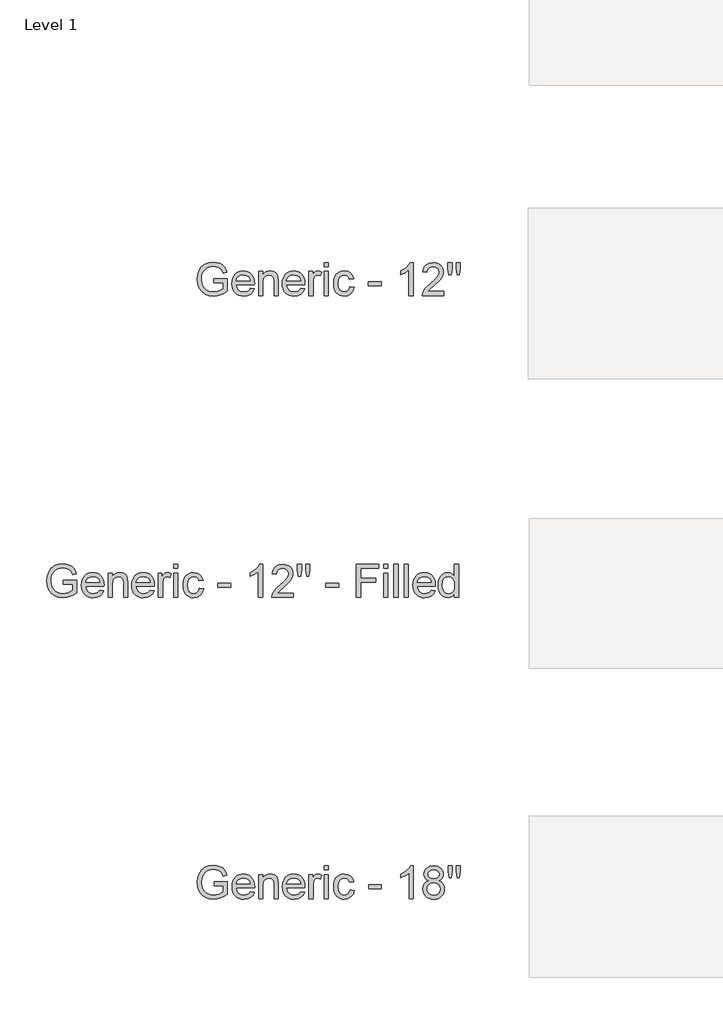
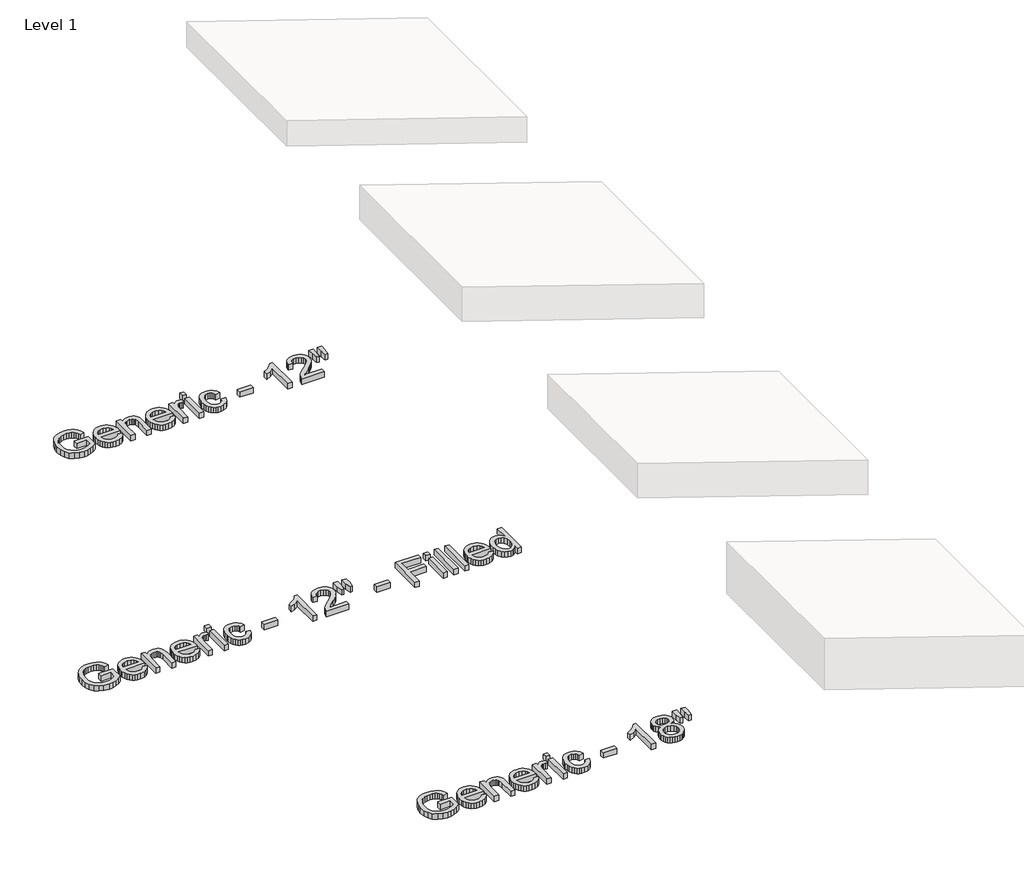
# One storey, part 4 of 42: 3 proxies.
"""IFC4 building model written with IfcOpenShell, lengths in millimetres."""

from ifc_helpers import new_model, si_unit, origin, origin_with_axes, place, context, project, spatial, polyline, outline, extrude, element, save

model = new_model("IFC4")

# Units and contexts
model_context = context("Model", 3, world=origin())
ifc_project = project(units=[si_unit("LENGTHUNIT", "METRE", prefix="MILLI")], contexts=[model_context])

# Site, building, storey
site = spatial("IfcSite", under=ifc_project)
building = spatial("IfcBuilding", under=site)
storey = spatial("IfcBuildingStorey", under=building, Name="Level 1", Elevation=0.0)

# Proxies
placement = place(None, origin())
element("IfcBuildingElementProxy", 1, Name="8\" Arial", ObjectType="8\" Arial", at=placement, inside=storey, context=model_context, shape_type="SweptSolid", body=[
    extrude(outline(polyline([(-15702.4339019, -8427.0985028), (-15702.4339019, -8389.027616), (-15578.7035199, -8389.027616), (-15578.7035199, -8502.8684903), (-15608.7717129, -8523.781453), (-15639.7879603, -8538.7830182), (-15671.6779047, -8547.8174181), (-15704.3671891, -8550.8288847), (-15747.0761063, -8546.0421399), (-15785.6767881, -8531.6819055), (-15817.7433309, -8508.2500927), (-15840.849831, -8476.2486124), (-15854.8196901, -8437.8617076), (-15859.4763098, -8395.2736209), (-15854.8382794, -8352.3788107), (-15840.9241882, -8312.4768779), (-15818.3103045, -8279.0068429), (-15803.9570411, -8265.9734198), (-15787.5728967, -8255.4077263), (-15750.1340461, -8241.4099833), (-15707.4158343, -8236.744069), (-15676.0556849, -8239.4488121), (-15647.8557166, -8247.5630417), (-15624.1078856, -8260.5011946), (-15606.1041484, -8277.6777079), (-15592.7849148, -8299.9198056), (-15583.0905948, -8328.0547114), (-15618.1871935, -8337.9442191), (-15626.0225835, -8317.8770696), (-15635.5495999, -8302.7360846), (-15648.1531454, -8291.3222543), (-15665.2181229, -8282.4365688), (-15685.564112, -8276.720359), (-15708.0106919, -8274.8149557), (-15734.2866677, -8276.8690734), (-15756.751837, -8283.0314264), (-15775.3225479, -8292.5305588), (-15789.9151485, -8304.5950146), (-15809.5082709, -8333.9289303), (-15818.431135, -8362.6679883), (-15821.405423, -8393.7121196), (-15817.8269827, -8430.119264), (-15807.0916619, -8460.0759213), (-15789.5247732, -8483.3683144), (-15765.4516295, -8499.7826664), (-15737.2795451, -8509.5141651), (-15707.4158343, -8512.757998), (-15681.046912, -8510.313505), (-15655.3286152, -8502.9800261), (-15632.9935711, -8492.8767414), (-15616.7744067, -8482.1228313), (-15616.7744067, -8427.0985028), (-15702.4339019, -8427.0985028)])), origin_with_axes(), (0.0, 0.0, 1.0), 50.8),
    extrude(outline(polyline([(-15365.0009251, -8479.445972), (-15327.6736104, -8484.2048329), (-15341.122969, -8512.3304441), (-15362.5843161, -8533.3549426), (-15391.5743297, -8546.4603992), (-15427.6096881, -8550.8288847), (-15451.2320413, -8548.9443944), (-15472.2797764, -8543.2909235), (-15490.7528935, -8533.868472), (-15506.6513924, -8520.6770398), (-15519.4361836, -8504.0837658), (-15528.5681773, -8484.4557884), (-15534.0473736, -8461.7931079), (-15535.8737723, -8436.095724), (-15534.0287843, -8409.5269668), (-15528.4938201, -8386.1090959), (-15519.2688799, -8365.8421114), (-15506.3539636, -8348.7260132), (-15490.4972906, -8335.1279401), (-15472.4470801, -8325.4150308), (-15452.2033322, -8319.5872852), (-15429.7660469, -8317.6447033), (-15408.0514206, -8319.5826379), (-15388.4141487, -8325.3964415), (-15370.854231, -8335.0861142), (-15355.3716676, -8348.651656), (-15342.7332672, -8365.7305756), (-15333.7058383, -8385.9603815), (-15328.2893809, -8409.3410738), (-15326.4838951, -8435.8726524), (-15326.7069667, -8446.1339461), (-15497.8028856, -8446.1339461), (-15491.2129786, -8474.6313433), (-15475.9046899, -8495.5814846), (-15453.8113067, -8508.4638696), (-15426.8661161, -8512.757998), (-15406.6037789, -8510.7689428), (-15389.5388013, -8504.8017775), (-15375.6711834, -8494.4847159), (-15365.0009251, -8479.445972)]), holes=[polyline([(-15497.8028856, -8408.0630594), (-15364.5547819, -8408.0630594), (-15369.704018, -8387.9494366), (-15379.798008, -8373.5613183), (-15401.9936325, -8360.1770221), (-15429.9147613, -8355.7155901), (-15455.5772902, -8359.2754411), (-15476.7969764, -8369.954994), (-15491.547586, -8386.6017123), (-15497.8028856, -8408.0630594)])]), origin_with_axes(), (0.0, 0.0, 1.0), 50.8),
    extrude(outline(polyline([(-15288.4130084, -8546.0700239), (-15288.4130084, -8322.4035642), (-15250.3421216, -8322.4035642), (-15250.3421216, -8353.6335885), (-15237.1158345, -8337.8884512), (-15221.2312775, -8326.6419246), (-15202.6884506, -8319.8940086), (-15181.4873538, -8317.6447033), (-15162.7214552, -8319.4571601), (-15145.5356472, -8324.8945304), (-15131.2032968, -8333.2783048), (-15120.997771, -8343.9299738), (-15109.5839407, -8371.9254598), (-15107.5762963, -8408.7322742), (-15107.5762963, -8546.0700239), (-15145.647183, -8546.0700239), (-15145.647183, -8413.862921), (-15150.0342579, -8380.1791091), (-15156.1036644, -8370.1501817), (-15165.5377342, -8362.3705595), (-15177.630074, -8357.3793324), (-15191.6742903, -8355.7155901), (-15213.9721558, -8359.4520394), (-15232.9797153, -8370.6613874), (-15240.575768, -8379.8119704), (-15246.00152, -8392.3179221), (-15250.3421216, -8427.3959316), (-15250.3421216, -8546.0700239), (-15288.4130084, -8546.0700239)])), origin_with_axes(), (0.0, 0.0, 1.0), 50.8),
    extrude(outline(polyline([(-14898.6325623, -8479.445972), (-14861.3052476, -8484.2048329), (-14874.7546062, -8512.3304441), (-14896.2159533, -8533.3549426), (-14925.2059669, -8546.4603992), (-14961.2413253, -8550.8288847), (-14984.8636785, -8548.9443944), (-15005.9114136, -8543.2909235), (-15024.3845307, -8533.868472), (-15040.2830296, -8520.6770398), (-15053.0678208, -8504.0837658), (-15062.1998146, -8484.4557884), (-15067.6790108, -8461.7931079), (-15069.5054095, -8436.095724), (-15067.6604215, -8409.5269668), (-15062.1254574, -8386.1090959), (-15052.9005171, -8365.8421114), (-15039.9856008, -8348.7260132), (-15024.1289278, -8335.1279401), (-15006.0787173, -8325.4150308), (-14985.8349694, -8319.5872852), (-14963.3976841, -8317.6447033), (-14941.6830579, -8319.5826379), (-14922.0457859, -8325.3964415), (-14904.4858682, -8335.0861142), (-14889.0033048, -8348.651656), (-14876.3649044, -8365.7305756), (-14867.3374755, -8385.9603815), (-14861.9210181, -8409.3410738), (-14860.1155323, -8435.8726524), (-14860.338604, -8446.1339461), (-15031.4345228, -8446.1339461), (-15024.8446158, -8474.6313433), (-15009.5363272, -8495.5814846), (-14987.4429439, -8508.4638696), (-14960.4977533, -8512.757998), (-14940.2354161, -8510.7689428), (-14923.1704385, -8504.8017775), (-14909.3028206, -8494.4847159), (-14898.6325623, -8479.445972)]), holes=[polyline([(-15031.4345228, -8408.0630594), (-14898.1864191, -8408.0630594), (-14903.3356553, -8387.9494366), (-14913.4296453, -8373.5613183), (-14935.6252697, -8360.1770221), (-14963.5463985, -8355.7155901), (-14989.2089274, -8359.2754411), (-15010.4286136, -8369.954994), (-15025.1792233, -8386.6017123), (-15031.4345228, -8408.0630594)])]), origin_with_axes(), (0.0, 0.0, 1.0), 50.8),
    extrude(outline(polyline([(-14822.0446456, -8546.0700239), (-14822.0446456, -8322.4035642), (-14788.7326197, -8322.4035642), (-14788.7326197, -8355.4925185), (-14776.426503, -8336.3083607), (-14765.0870299, -8325.0060662), (-14753.7103781, -8319.485044), (-14741.2927256, -8317.6447033), (-14722.3316395, -8320.5818128), (-14703.0731245, -8329.393141), (-14715.7882058, -8363.5230962), (-14729.1725019, -8357.6674666), (-14742.556798, -8355.7155901), (-14753.9241551, -8357.5931094), (-14764.0832076, -8363.2256674), (-14772.2903837, -8372.18571), (-14777.8021112, -8384.0456835), (-14782.4308469, -8405.3118429), (-14783.9737588, -8428.5112896), (-14783.9737588, -8546.0700239), (-14822.0446456, -8546.0700239)])), origin_with_axes(), (0.0, 0.0, 1.0), 50.8),
    extrude(outline(polyline([(-14679.2788202, -8279.5738166), (-14679.2788202, -8241.5029298), (-14641.2079335, -8241.5029298), (-14641.2079335, -8279.5738166), (-14679.2788202, -8279.5738166)])), origin_with_axes(), (0.0, 0.0, 1.0), 50.8),
    extrude(outline(polyline([(-14679.2788202, -8546.0700239), (-14679.2788202, -8322.4035642), (-14641.2079335, -8322.4035642), (-14641.2079335, -8546.0700239), (-14679.2788202, -8546.0700239)])), origin_with_axes(), (0.0, 0.0, 1.0), 50.8),
    extrude(outline(polyline([(-14441.335778, -8465.1693895), (-14403.2648912, -8469.9282504), (-14413.8793816, -8503.7886606), (-14433.8257007, -8529.3768323), (-14461.2263292, -8545.4658716), (-14494.2037477, -8550.8288847), (-14515.5558826, -8548.9583364), (-14534.7005381, -8543.3466914), (-14551.6377143, -8533.9939497), (-14566.367411, -8520.9001114), (-14578.2901234, -8504.3114847), (-14586.8063465, -8484.4743777), (-14591.9160804, -8461.3887906), (-14593.619325, -8435.0547232), (-14590.7100996, -8401.1757237), (-14581.9824231, -8371.813924), (-14567.296876, -8348.1032717), (-14546.5140384, -8331.1777139), (-14521.6508494, -8321.027956), (-14494.7242481, -8317.6447033), (-14462.5554642, -8322.2920284), (-14436.8371674, -8336.2340035), (-14418.3872869, -8358.7270567), (-14408.0237521, -8389.027616), (-14446.0946388, -8393.7864768), (-14453.0005639, -8377.1769371), (-14463.754474, -8365.2704904), (-14477.7615117, -8358.1043152), (-14494.4268193, -8355.7155901), (-14519.0297581, -8360.418683), (-14538.5578179, -8374.5279619), (-14551.3007832, -8398.8055879), (-14555.5484383, -8434.0137224), (-14551.3937297, -8469.6958841), (-14538.9296039, -8494.057162), (-14519.7547408, -8508.082789), (-14495.4678201, -8512.757998), (-14475.7538673, -8509.8394778), (-14459.5904708, -8501.0839175), (-14447.8327384, -8486.2682452), (-14441.335778, -8465.1693895)])), origin_with_axes(), (0.0, 0.0, 1.0), 50.8),
    extrude(outline(polyline([(-14270.0167876, -8455.6516678), (-14270.0167876, -8417.5807811), (-14151.0452665, -8417.5807811), (-14151.0452665, -8455.6516678), (-14270.0167876, -8455.6516678)])), origin_with_axes(), (0.0, 0.0, 1.0), 50.8),
    extrude(outline(polyline([(-13855.9958941, -8546.0700239), (-13894.0667809, -8546.0700239), (-13894.0667809, -8308.7218392), (-13930.1300232, -8334.4122521), (-13970.2085544, -8353.6335885), (-13970.2085544, -8317.6447033), (-13940.307665, -8301.3790657), (-13914.4034752, -8282.0276042), (-13893.983129, -8261.4492489), (-13880.5337703, -8241.5029298), (-13855.9958941, -8241.5029298), (-13855.9958941, -8546.0700239)])), origin_with_axes(), (0.0, 0.0, 1.0), 50.8),
    extrude(outline(polyline([(-13570.4642434, -8507.9991371), (-13570.4642434, -8546.0700239), (-13770.3363989, -8546.0700239), (-13766.2467528, -8519.821932), (-13756.8591563, -8499.3086393), (-13743.1216634, -8479.4087934), (-13723.2497015, -8458.5794826), (-13695.4586978, -8435.2777948), (-13654.3763444, -8398.7869986), (-13629.7269324, -8371.8511026), (-13617.4022263, -8349.9900856), (-13613.293991, -8328.7239262), (-13617.1698601, -8309.6605989), (-13628.7974674, -8293.8132205), (-13646.6710795, -8283.1336675), (-13669.2849631, -8279.5738166), (-13693.0327941, -8283.0500157), (-13711.4826745, -8293.4786131), (-13723.3891213, -8310.0416796), (-13727.5066513, -8331.9212859), (-13765.577538, -8327.162425), (-13762.3034975, -8307.5088874), (-13756.3479505, -8290.3370214), (-13747.7108969, -8275.6468269), (-13736.3923368, -8263.438304), (-13722.6525203, -8253.8415778), (-13706.7516976, -8246.9867734), (-13668.4670339, -8241.5029298), (-13648.0629533, -8243.0272524), (-13629.9035307, -8247.6002203), (-13613.9887661, -8255.2218333), (-13600.3186595, -8265.8920916), (-13589.3393541, -8278.8209499), (-13581.4969931, -8293.2183629), (-13576.7915764, -8309.0843306), (-13575.2231042, -8326.418853), (-13576.9147306, -8344.6270725), (-13581.9896095, -8362.5192739), (-13590.9961254, -8380.7181988), (-13604.4826627, -8399.8465887), (-13625.9811884, -8422.683544), (-13659.0236694, -8452.008165), (-13702.8200606, -8488.6290863), (-13719.996574, -8507.9991371), (-13570.4642434, -8507.9991371)])), origin_with_axes(), (0.0, 0.0, 1.0), 50.8),
    extrude(outline(polyline([(-13523.0987066, -8350.9567292), (-13532.3933566, -8292.1401835), (-13532.3933566, -8241.5029298), (-13494.3224699, -8241.5029298), (-13494.3224699, -8292.1401835), (-13502.6504764, -8350.9567292), (-13523.0987066, -8350.9567292)])), origin_with_axes(), (0.0, 0.0, 1.0), 50.8),
    extrude(outline(polyline([(-13447.1800046, -8350.9567292), (-13456.2515831, -8292.1401835), (-13456.2515831, -8241.5029298), (-13418.1806964, -8241.5029298), (-13418.1806964, -8292.1401835), (-13427.1035605, -8350.9567292), (-13447.1800046, -8350.9567292)])), origin_with_axes(), (0.0, 0.0, 1.0), 50.8),
])
element("IfcBuildingElementProxy", 2, Name="8\" Arial", ObjectType="8\" Arial", at=placement, inside=storey, context=model_context, shape_type="SweptSolid", body=[
    extrude(outline(polyline([(-17098.2012997, -11224.4993034), (-17098.2012997, -11186.4284167), (-16974.4709177, -11186.4284167), (-16974.4709177, -11300.2692909), (-17004.5391107, -11321.1822536), (-17035.5553581, -11336.1838189), (-17067.4453025, -11345.2182188), (-17100.1345869, -11348.2296854), (-17142.843504, -11343.4429406), (-17181.4441859, -11329.0827062), (-17213.5107287, -11305.6508933), (-17236.6172288, -11273.6494131), (-17250.5870879, -11235.2625082), (-17255.2437075, -11192.6744215), (-17250.6056772, -11149.7796114), (-17236.691586, -11109.8776785), (-17214.0777023, -11076.4076436), (-17199.7244389, -11063.3742205), (-17183.3402945, -11052.808527), (-17145.9014439, -11038.810784), (-17103.1832321, -11034.1448696), (-17071.8230827, -11036.8496128), (-17043.6231144, -11044.9638423), (-17019.8752834, -11057.9019952), (-17001.8715462, -11075.0785086), (-16988.5523126, -11097.3206063), (-16978.8579925, -11125.4555121), (-17013.9545913, -11135.3450198), (-17021.7899813, -11115.2778702), (-17031.3169976, -11100.1368852), (-17043.9205432, -11088.7230549), (-17060.9855207, -11079.8373695), (-17081.3315098, -11074.1211597), (-17103.7780897, -11072.2157564), (-17130.0540655, -11074.2698741), (-17152.5192348, -11080.4322271), (-17171.0899457, -11089.9313595), (-17185.6825463, -11101.9958153), (-17205.2756687, -11131.3297309), (-17214.1985328, -11160.068789), (-17217.1728208, -11191.1129203), (-17213.5943805, -11227.5200647), (-17202.8590597, -11257.4767219), (-17185.292171, -11280.769115), (-17161.2190273, -11297.1834671), (-17133.0469428, -11306.9149657), (-17103.1832321, -11310.1587986), (-17076.8143098, -11307.7143057), (-17051.096013, -11300.3808267), (-17028.7609689, -11290.2775421), (-17012.5418045, -11279.5236319), (-17012.5418045, -11224.4993034), (-17098.2012997, -11224.4993034)])), origin_with_axes(), (0.0, 0.0, 1.0), 50.8),
    extrude(outline(polyline([(-16760.7683229, -11276.8467727), (-16723.4410081, -11281.6056336), (-16736.8903668, -11309.7312447), (-16758.3517139, -11330.7557432), (-16787.3417275, -11343.8611998), (-16823.3770859, -11348.2296854), (-16846.9994391, -11346.3451951), (-16868.0471742, -11340.6917242), (-16886.5202912, -11331.2692726), (-16902.4187902, -11318.0778405), (-16915.2035814, -11301.4845664), (-16924.3355751, -11281.8565891), (-16929.8147714, -11259.1939085), (-16931.6411701, -11233.4965247), (-16929.7961821, -11206.9277674), (-16924.2612179, -11183.5098965), (-16915.0362777, -11163.242912), (-16902.1213614, -11146.1268139), (-16886.2646884, -11132.5287408), (-16868.2144779, -11122.8158315), (-16847.97073, -11116.9880859), (-16825.5334447, -11115.045504), (-16803.8188184, -11116.9834385), (-16784.1815465, -11122.7972422), (-16766.6216288, -11132.4869149), (-16751.1390654, -11146.0524567), (-16738.5006649, -11163.1313762), (-16729.473236, -11183.3611821), (-16724.0567787, -11206.7418744), (-16722.2512929, -11233.2734531), (-16722.4743645, -11243.5347468), (-16893.5702833, -11243.5347468), (-16886.9803764, -11272.032144), (-16871.6720877, -11292.9822853), (-16849.5787045, -11305.8646703), (-16822.6335139, -11310.1587986), (-16802.3711767, -11308.1697435), (-16785.3061991, -11302.2025782), (-16771.4385812, -11291.8855166), (-16760.7683229, -11276.8467727)]), holes=[polyline([(-16893.5702833, -11205.46386), (-16760.3221797, -11205.46386), (-16765.4714158, -11185.3502373), (-16775.5654058, -11170.9621189), (-16797.7610302, -11157.5778228), (-16825.6821591, -11153.1163907), (-16851.344688, -11156.6762417), (-16872.5643741, -11167.3557947), (-16887.3149838, -11184.002513), (-16893.5702833, -11205.46386)])]), origin_with_axes(), (0.0, 0.0, 1.0), 50.8),
    extrude(outline(polyline([(-16684.1804062, -11343.4708245), (-16684.1804062, -11119.8043648), (-16646.1095194, -11119.8043648), (-16646.1095194, -11151.0343891), (-16632.8832323, -11135.2892519), (-16616.9986753, -11124.0427253), (-16598.4558484, -11117.2948093), (-16577.2547516, -11115.045504), (-16558.488853, -11116.8579608), (-16541.303045, -11122.2953311), (-16526.9706946, -11130.6791054), (-16516.7651688, -11141.3307744), (-16505.3513385, -11169.3262605), (-16503.3436941, -11206.1330748), (-16503.3436941, -11343.4708245), (-16541.4145808, -11343.4708245), (-16541.4145808, -11211.2637217), (-16545.8016557, -11177.5799098), (-16551.8710622, -11167.5509823), (-16561.305132, -11159.7713602), (-16573.3974718, -11154.7801331), (-16587.4416881, -11153.1163907), (-16609.7395536, -11156.8528401), (-16628.747113, -11168.0621881), (-16636.3431658, -11177.2127711), (-16641.7689178, -11189.7187228), (-16646.1095194, -11224.7967322), (-16646.1095194, -11343.4708245), (-16684.1804062, -11343.4708245)])), origin_with_axes(), (0.0, 0.0, 1.0), 50.8),
    extrude(outline(polyline([(-16294.3999601, -11276.8467727), (-16257.0726453, -11281.6056336), (-16270.522004, -11309.7312447), (-16291.9833511, -11330.7557432), (-16320.9733647, -11343.8611998), (-16357.0087231, -11348.2296854), (-16380.6310763, -11346.3451951), (-16401.6788114, -11340.6917242), (-16420.1519285, -11331.2692726), (-16436.0504274, -11318.0778405), (-16448.8352186, -11301.4845664), (-16457.9672123, -11281.8565891), (-16463.4464086, -11259.1939085), (-16465.2728073, -11233.4965247), (-16463.4278193, -11206.9277674), (-16457.8928551, -11183.5098965), (-16448.6679149, -11163.242912), (-16435.7529986, -11146.1268139), (-16419.8963256, -11132.5287408), (-16401.8461151, -11122.8158315), (-16381.6023672, -11116.9880859), (-16359.1650819, -11115.045504), (-16337.4504556, -11116.9834385), (-16317.8131837, -11122.7972422), (-16300.253266, -11132.4869149), (-16284.7707026, -11146.0524567), (-16272.1323021, -11163.1313762), (-16263.1048733, -11183.3611821), (-16257.6884159, -11206.7418744), (-16255.8829301, -11233.2734531), (-16256.1060017, -11243.5347468), (-16427.2019205, -11243.5347468), (-16420.6120136, -11272.032144), (-16405.3037249, -11292.9822853), (-16383.2103417, -11305.8646703), (-16356.2651511, -11310.1587986), (-16336.0028139, -11308.1697435), (-16318.9378363, -11302.2025782), (-16305.0702184, -11291.8855166), (-16294.3999601, -11276.8467727)]), holes=[polyline([(-16427.2019205, -11205.46386), (-16293.9538169, -11205.46386), (-16299.103053, -11185.3502373), (-16309.197043, -11170.9621189), (-16331.3926674, -11157.5778228), (-16359.3137963, -11153.1163907), (-16384.9763252, -11156.6762417), (-16406.1960113, -11167.3557947), (-16420.946621, -11184.002513), (-16427.2019205, -11205.46386)])]), origin_with_axes(), (0.0, 0.0, 1.0), 50.8),
    extrude(outline(polyline([(-16217.8120434, -11343.4708245), (-16217.8120434, -11119.8043648), (-16184.5000175, -11119.8043648), (-16184.5000175, -11152.8933191), (-16172.1939007, -11133.7091614), (-16160.8544276, -11122.4068669), (-16149.4777759, -11116.8858447), (-16137.0601234, -11115.045504), (-16118.0990372, -11117.9826134), (-16098.8405223, -11126.7939417), (-16111.5556036, -11160.9238968), (-16124.9398997, -11155.0682673), (-16138.3241958, -11153.1163907), (-16149.6915529, -11154.9939101), (-16159.8506054, -11160.626468), (-16168.0577815, -11169.5865107), (-16173.569509, -11181.4464842), (-16178.1982447, -11202.7126436), (-16179.7411566, -11225.9120902), (-16179.7411566, -11343.4708245), (-16217.8120434, -11343.4708245)])), origin_with_axes(), (0.0, 0.0, 1.0), 50.8),
    extrude(outline(polyline([(-16075.046218, -11076.9746172), (-16075.046218, -11038.9037305), (-16036.9753313, -11038.9037305), (-16036.9753313, -11076.9746172), (-16075.046218, -11076.9746172)])), origin_with_axes(), (0.0, 0.0, 1.0), 50.8),
    extrude(outline(polyline([(-16075.046218, -11343.4708245), (-16075.046218, -11119.8043648), (-16036.9753313, -11119.8043648), (-16036.9753313, -11343.4708245), (-16075.046218, -11343.4708245)])), origin_with_axes(), (0.0, 0.0, 1.0), 50.8),
    extrude(outline(polyline([(-15837.1031758, -11262.5701902), (-15799.032289, -11267.329051), (-15809.6467794, -11301.1894613), (-15829.5930985, -11326.777633), (-15856.993727, -11342.8666723), (-15889.9711455, -11348.2296854), (-15911.3232804, -11346.3591371), (-15930.4679359, -11340.7474921), (-15947.405112, -11331.3947504), (-15962.1348088, -11318.3009121), (-15974.0575212, -11301.7122854), (-15982.5737443, -11281.8751784), (-15987.6834782, -11258.7895913), (-15989.3867228, -11232.4555239), (-15986.4774973, -11198.5765243), (-15977.7498209, -11169.2147247), (-15963.0642738, -11145.5040723), (-15942.2814362, -11128.5785145), (-15917.4182472, -11118.4287566), (-15890.4916459, -11115.045504), (-15858.3228619, -11119.692829), (-15832.6045651, -11133.6348042), (-15814.1546847, -11156.1278574), (-15803.7911499, -11186.4284167), (-15841.8620366, -11191.1872775), (-15848.7679616, -11174.5777378), (-15859.5218718, -11162.671291), (-15873.5289095, -11155.5051158), (-15890.1942171, -11153.1163907), (-15914.7971559, -11157.8194837), (-15934.3252157, -11171.9287625), (-15947.068181, -11196.2063886), (-15951.3158361, -11231.4145231), (-15947.1611275, -11267.0966848), (-15934.6970017, -11291.4579626), (-15915.5221386, -11305.4835896), (-15891.2352179, -11310.1587986), (-15871.5212651, -11307.2402785), (-15855.3578686, -11298.4847181), (-15843.6001362, -11283.6690459), (-15837.1031758, -11262.5701902)])), origin_with_axes(), (0.0, 0.0, 1.0), 50.8),
    extrude(outline(polyline([(-15665.7841854, -11253.0524685), (-15665.7841854, -11214.9815817), (-15546.8126643, -11214.9815817), (-15546.8126643, -11253.0524685), (-15665.7841854, -11253.0524685)])), origin_with_axes(), (0.0, 0.0, 1.0), 50.8),
    extrude(outline(polyline([(-15251.7632919, -11343.4708245), (-15289.8341786, -11343.4708245), (-15289.8341786, -11106.1226399), (-15325.897421, -11131.8130527), (-15365.9759522, -11151.0343891), (-15365.9759522, -11115.045504), (-15336.0750628, -11098.7798663), (-15310.170873, -11079.4284049), (-15289.7505268, -11058.8500496), (-15276.3011681, -11038.9037305), (-15251.7632919, -11038.9037305), (-15251.7632919, -11343.4708245)])), origin_with_axes(), (0.0, 0.0, 1.0), 50.8),
    extrude(outline(polyline([(-14966.2316412, -11305.3999378), (-14966.2316412, -11343.4708245), (-15166.1037967, -11343.4708245), (-15162.0141506, -11317.2227327), (-15152.626554, -11296.7094399), (-15138.8890612, -11276.8095941), (-15119.0170993, -11255.9802833), (-15091.2260956, -11232.6785955), (-15050.1437422, -11196.1877993), (-15025.4943301, -11169.2519033), (-15013.1696241, -11147.3908863), (-15009.0613888, -11126.1247269), (-15012.9372579, -11107.0613996), (-15024.5648651, -11091.2140212), (-15042.4384773, -11080.5344682), (-15065.0523609, -11076.9746172), (-15088.8001919, -11080.4508164), (-15107.2500723, -11090.8794138), (-15119.1565191, -11107.4424802), (-15123.2740491, -11129.3220865), (-15161.3449358, -11124.5632257), (-15158.0708953, -11104.9096881), (-15152.1153483, -11087.737822), (-15143.4782947, -11073.0476276), (-15132.1597346, -11060.8391047), (-15118.4199181, -11051.2423785), (-15102.5190954, -11044.387574), (-15064.2344317, -11038.9037305), (-15043.8303511, -11040.4280531), (-15025.6709285, -11045.0010209), (-15009.7561639, -11052.622634), (-14996.0860573, -11063.2928923), (-14985.1067519, -11076.2217506), (-14977.2643908, -11090.6191636), (-14972.5589742, -11106.4851313), (-14970.990502, -11123.8196537), (-14972.6821283, -11142.0278732), (-14977.7570073, -11159.9200746), (-14986.7635232, -11178.1189995), (-15000.2500605, -11197.2473894), (-15021.7485862, -11220.0843446), (-15054.7910672, -11249.4089657), (-15098.5874584, -11286.029887), (-15115.7639718, -11305.3999378), (-14966.2316412, -11305.3999378)])), origin_with_axes(), (0.0, 0.0, 1.0), 50.8),
    extrude(outline(polyline([(-14918.8661043, -11148.3575299), (-14928.1607544, -11089.5409841), (-14928.1607544, -11038.9037305), (-14890.0898677, -11038.9037305), (-14890.0898677, -11089.5409841), (-14898.4178741, -11148.3575299), (-14918.8661043, -11148.3575299)])), origin_with_axes(), (0.0, 0.0, 1.0), 50.8),
    extrude(outline(polyline([(-14842.9474024, -11148.3575299), (-14852.0189809, -11089.5409841), (-14852.0189809, -11038.9037305), (-14813.9480942, -11038.9037305), (-14813.9480942, -11089.5409841), (-14822.8709582, -11148.3575299), (-14842.9474024, -11148.3575299)])), origin_with_axes(), (0.0, 0.0, 1.0), 50.8),
    extrude(outline(polyline([(-14666.423408, -11253.0524685), (-14666.423408, -11214.9815817), (-14547.4518868, -11214.9815817), (-14547.4518868, -11253.0524685), (-14666.423408, -11253.0524685)])), origin_with_axes(), (0.0, 0.0, 1.0), 50.8),
    extrude(outline(polyline([(-14380.8917573, -11343.4708245), (-14380.8917573, -11038.9037305), (-14176.2607409, -11038.9037305), (-14176.2607409, -11076.9746172), (-14342.8208705, -11076.9746172), (-14342.8208705, -11167.3929733), (-14200.0550452, -11167.3929733), (-14200.0550452, -11205.46386), (-14342.8208705, -11205.46386), (-14342.8208705, -11343.4708245), (-14380.8917573, -11343.4708245)])), origin_with_axes(), (0.0, 0.0, 1.0), 50.8),
    extrude(outline(polyline([(-14128.6721325, -11076.9746172), (-14128.6721325, -11038.9037305), (-14090.6012457, -11038.9037305), (-14090.6012457, -11076.9746172), (-14128.6721325, -11076.9746172)])), origin_with_axes(), (0.0, 0.0, 1.0), 50.8),
    extrude(outline(polyline([(-14128.6721325, -11343.4708245), (-14128.6721325, -11119.8043648), (-14090.6012457, -11119.8043648), (-14090.6012457, -11343.4708245), (-14128.6721325, -11343.4708245)])), origin_with_axes(), (0.0, 0.0, 1.0), 50.8),
    extrude(outline(polyline([(-14033.4949156, -11343.4708245), (-14033.4949156, -11038.9037305), (-13995.4240288, -11038.9037305), (-13995.4240288, -11343.4708245), (-14033.4949156, -11343.4708245)])), origin_with_axes(), (0.0, 0.0, 1.0), 50.8),
    extrude(outline(polyline([(-13938.3176987, -11343.4708245), (-13938.3176987, -11038.9037305), (-13900.2468119, -11038.9037305), (-13900.2468119, -11343.4708245), (-13938.3176987, -11343.4708245)])), origin_with_axes(), (0.0, 0.0, 1.0), 50.8),
    extrude(outline(polyline([(-13686.5442171, -11276.8467727), (-13649.2169024, -11281.6056336), (-13662.6662611, -11309.7312447), (-13684.1276081, -11330.7557432), (-13713.1176217, -11343.8611998), (-13749.1529801, -11348.2296854), (-13772.7753333, -11346.3451951), (-13793.8230684, -11340.6917242), (-13812.2961855, -11331.2692726), (-13828.1946845, -11318.0778405), (-13840.9794757, -11301.4845664), (-13850.1114694, -11281.8565891), (-13855.5906656, -11259.1939085), (-13857.4170643, -11233.4965247), (-13855.5720763, -11206.9277674), (-13850.0371122, -11183.5098965), (-13840.812172, -11163.242912), (-13827.8972557, -11146.1268139), (-13812.0405826, -11132.5287408), (-13793.9903721, -11122.8158315), (-13773.7466243, -11116.9880859), (-13751.3093389, -11115.045504), (-13729.5947127, -11116.9834385), (-13709.9574407, -11122.7972422), (-13692.397523, -11132.4869149), (-13676.9149596, -11146.0524567), (-13664.2765592, -11163.1313762), (-13655.2491303, -11183.3611821), (-13649.832673, -11206.7418744), (-13648.0271872, -11233.2734531), (-13648.2502588, -11243.5347468), (-13819.3461776, -11243.5347468), (-13812.7562707, -11272.032144), (-13797.447982, -11292.9822853), (-13775.3545987, -11305.8646703), (-13748.4094081, -11310.1587986), (-13728.1470709, -11308.1697435), (-13711.0820934, -11302.2025782), (-13697.2144754, -11291.8855166), (-13686.5442171, -11276.8467727)]), holes=[polyline([(-13819.3461776, -11205.46386), (-13686.0980739, -11205.46386), (-13691.2473101, -11185.3502373), (-13701.3413001, -11170.9621189), (-13723.5369245, -11157.5778228), (-13751.4580533, -11153.1163907), (-13777.1205822, -11156.6762417), (-13798.3402684, -11167.3557947), (-13813.0908781, -11184.002513), (-13819.3461776, -11205.46386)])]), origin_with_axes(), (0.0, 0.0, 1.0), 50.8),
    extrude(outline(polyline([(-13471.9493359, -11343.4708245), (-13471.9493359, -11307.5562966), (-13483.3399296, -11325.3509042), (-13497.1378377, -11338.0613382), (-13513.3430601, -11345.6875986), (-13531.9555969, -11348.2296854), (-13556.5678303, -11344.5490039), (-13579.0980621, -11333.5069596), (-13598.1706841, -11315.8750084), (-13612.410088, -11292.4246063), (-13621.2771842, -11264.1038074), (-13624.2328829, -11231.8606663), (-13621.5095505, -11200.0171951), (-13613.339553, -11171.2595477), (-13599.7321853, -11147.2235826), (-13580.6967419, -11129.5451581), (-13557.6738937, -11118.6704175), (-13532.1043113, -11115.045504), (-13513.4778325, -11117.6387114), (-13497.0077126, -11125.4183335), (-13483.0471481, -11137.3433695), (-13471.9493359, -11152.3728187), (-13471.9493359, -11038.9037305), (-13433.8784492, -11038.9037305), (-13433.8784492, -11343.4708245), (-13471.9493359, -11343.4708245)]), holes=[polyline([(-13586.1619962, -11231.7119519), (-13581.8678679, -11266.1486305), (-13568.9854828, -11290.6400334), (-13550.2660576, -11305.2791073), (-13528.4608084, -11310.1587986), (-13506.664854, -11305.5021789), (-13488.4194559, -11291.5323199), (-13476.0668659, -11267.9889712), (-13471.9493359, -11234.6118827), (-13476.1412231, -11198.1210865), (-13488.7168847, -11172.8210489), (-13507.4270153, -11158.0425553), (-13530.0223097, -11153.1163907), (-13552.0506304, -11157.8473676), (-13570.1008408, -11172.0402983), (-13582.1467074, -11196.4201655), (-13586.1619962, -11231.7119519)])]), origin_with_axes(), (0.0, 0.0, 1.0), 50.8),
])
element("IfcBuildingElementProxy", 3, Name="8\" Arial", ObjectType="8\" Arial", at=placement, inside=storey, context=model_context, shape_type="SweptSolid", body=[
    extrude(outline(polyline([(-15701.6648928, -14020.780444), (-15701.6648928, -13982.7095572), (-15577.9345108, -13982.7095572), (-15577.9345108, -14096.5504315), (-15608.0027038, -14117.4633942), (-15639.0189512, -14132.4649594), (-15670.9088956, -14141.4993593), (-15703.59818, -14144.510826), (-15746.3070971, -14139.7240812), (-15784.907779, -14125.3638468), (-15816.9743218, -14101.9320339), (-15840.0808219, -14069.9305537), (-15854.050681, -14031.5436488), (-15858.7073007, -13988.9555621), (-15854.0692703, -13946.0607519), (-15840.1551791, -13906.1588191), (-15817.5412954, -13872.6887842), (-15803.188032, -13859.6553611), (-15786.8038876, -13849.0896676), (-15749.365037, -13835.0919245), (-15706.6468252, -13830.4260102), (-15675.2866758, -13833.1307534), (-15647.0867075, -13841.2449829), (-15623.3388765, -13854.1831358), (-15605.3351393, -13871.3596492), (-15592.0159057, -13893.6017468), (-15582.3215857, -13921.7366527), (-15617.4181844, -13931.6261604), (-15625.2535744, -13911.5590108), (-15634.7805907, -13896.4180258), (-15647.3841363, -13885.0041955), (-15664.4491138, -13876.11851), (-15684.7951029, -13870.4023002), (-15707.2416828, -13868.496897), (-15733.5176586, -13870.5510146), (-15755.9828279, -13876.7133676), (-15774.5535388, -13886.2125), (-15789.1461394, -13898.2769558), (-15808.7392618, -13927.6108715), (-15817.6621259, -13956.3499296), (-15820.6364139, -13987.3940609), (-15817.0579736, -14023.8012053), (-15806.3226528, -14053.7578625), (-15788.7557641, -14077.0502556), (-15764.6826204, -14093.4646077), (-15736.510536, -14103.1961063), (-15706.6468252, -14106.4399392), (-15680.2779029, -14103.9954462), (-15654.5596061, -14096.6619673), (-15632.224562, -14086.5586827), (-15616.0053976, -14075.8047725), (-15616.0053976, -14020.780444), (-15701.6648928, -14020.780444)])), origin_with_axes(), (0.0, 0.0, 1.0), 50.8),
    extrude(outline(polyline([(-15364.231916, -14073.1279133), (-15326.9046012, -14077.8867741), (-15340.3539599, -14106.0123853), (-15361.815307, -14127.0368838), (-15390.8053206, -14140.1423404), (-15426.840679, -14144.510826), (-15450.4630322, -14142.6263357), (-15471.5107673, -14136.9728647), (-15489.9838844, -14127.5504132), (-15505.8823833, -14114.3589811), (-15518.6671745, -14097.765707), (-15527.7991682, -14078.1377297), (-15533.2783645, -14055.4750491), (-15535.1047632, -14029.7776653), (-15533.2597752, -14003.208908), (-15527.724811, -13979.7910371), (-15518.4998708, -13959.5240526), (-15505.5849545, -13942.4079545), (-15489.7282815, -13928.8098814), (-15471.678071, -13919.096972), (-15451.4343231, -13913.2692264), (-15428.9970378, -13911.3266446), (-15407.2824115, -13913.2645791), (-15387.6451396, -13919.0783827), (-15370.0852219, -13928.7680555), (-15354.6026585, -13942.3335973), (-15341.9642581, -13959.4125168), (-15332.9368292, -13979.6423227), (-15327.5203718, -14003.023015), (-15325.714886, -14029.5545937), (-15325.9379576, -14039.8158874), (-15497.0338765, -14039.8158874), (-15490.4439695, -14068.3132845), (-15475.1356808, -14089.2634258), (-15453.0422976, -14102.1458109), (-15426.097107, -14106.4399392), (-15405.8347698, -14104.4508841), (-15388.7697922, -14098.4837187), (-15374.9021743, -14088.1666571), (-15364.231916, -14073.1279133)]), holes=[polyline([(-15497.0338765, -14001.7450006), (-15363.7857728, -14001.7450006), (-15368.9350089, -13981.6313778), (-15379.0289989, -13967.2432595), (-15401.2246233, -13953.8589634), (-15429.1457522, -13949.3975313), (-15454.8082811, -13952.9573823), (-15476.0279673, -13963.6369353), (-15490.7785769, -13980.2836536), (-15497.0338765, -14001.7450006)])]), origin_with_axes(), (0.0, 0.0, 1.0), 50.8),
    extrude(outline(polyline([(-15287.6439993, -14139.7519651), (-15287.6439993, -13916.0855054), (-15249.5731125, -13916.0855054), (-15249.5731125, -13947.3155297), (-15236.3468254, -13931.5703925), (-15220.4622684, -13920.3238658), (-15201.9194415, -13913.5759499), (-15180.7183447, -13911.3266446), (-15161.9524461, -13913.1391013), (-15144.7666381, -13918.5764716), (-15130.4342877, -13926.960246), (-15120.2287619, -13937.611915), (-15108.8149316, -13965.6074011), (-15106.8072872, -14002.4142154), (-15106.8072872, -14139.7519651), (-15144.8781739, -14139.7519651), (-15144.8781739, -14007.5448623), (-15149.2652488, -13973.8610504), (-15155.3346553, -13963.8321229), (-15164.7687251, -13956.0525008), (-15176.8610649, -13951.0612737), (-15190.9052812, -13949.3975313), (-15213.2031467, -13953.1339807), (-15232.2107062, -13964.3433287), (-15239.8067589, -13973.4939117), (-15245.2325109, -13985.9998634), (-15249.5731125, -14021.0778728), (-15249.5731125, -14139.7519651), (-15287.6439993, -14139.7519651)])), origin_with_axes(), (0.0, 0.0, 1.0), 50.8),
    extrude(outline(polyline([(-14897.8635532, -14073.1279133), (-14860.5362385, -14077.8867741), (-14873.9855971, -14106.0123853), (-14895.4469442, -14127.0368838), (-14924.4369578, -14140.1423404), (-14960.4723162, -14144.510826), (-14984.0946694, -14142.6263357), (-15005.1424045, -14136.9728647), (-15023.6155216, -14127.5504132), (-15039.5140205, -14114.3589811), (-15052.2988117, -14097.765707), (-15061.4308054, -14078.1377297), (-15066.9100017, -14055.4750491), (-15068.7364004, -14029.7776653), (-15066.8914124, -14003.208908), (-15061.3564482, -13979.7910371), (-15052.131508, -13959.5240526), (-15039.2165917, -13942.4079545), (-15023.3599187, -13928.8098814), (-15005.3097082, -13919.096972), (-14985.0659603, -13913.2692264), (-14962.628675, -13911.3266446), (-14940.9140488, -13913.2645791), (-14921.2767768, -13919.0783827), (-14903.7168591, -13928.7680555), (-14888.2342957, -13942.3335973), (-14875.5958953, -13959.4125168), (-14866.5684664, -13979.6423227), (-14861.152009, -14003.023015), (-14859.3465232, -14029.5545937), (-14859.5695948, -14039.8158874), (-15030.6655137, -14039.8158874), (-15024.0756067, -14068.3132845), (-15008.7673181, -14089.2634258), (-14986.6739348, -14102.1458109), (-14959.7287442, -14106.4399392), (-14939.466407, -14104.4508841), (-14922.4014294, -14098.4837187), (-14908.5338115, -14088.1666571), (-14897.8635532, -14073.1279133)]), holes=[polyline([(-15030.6655137, -14001.7450006), (-14897.41741, -14001.7450006), (-14902.5666462, -13981.6313778), (-14912.6606361, -13967.2432595), (-14934.8562606, -13953.8589634), (-14962.7773894, -13949.3975313), (-14988.4399183, -13952.9573823), (-15009.6596045, -13963.6369353), (-15024.4102142, -13980.2836536), (-15030.6655137, -14001.7450006)])]), origin_with_axes(), (0.0, 0.0, 1.0), 50.8),
    extrude(outline(polyline([(-14821.2756365, -14139.7519651), (-14821.2756365, -13916.0855054), (-14787.9636106, -13916.0855054), (-14787.9636106, -13949.1744597), (-14775.6574939, -13929.9903019), (-14764.3180208, -13918.6880074), (-14752.941369, -13913.1669853), (-14740.5237165, -13911.3266446), (-14721.5626303, -13914.263754), (-14702.3041154, -13923.0750823), (-14715.0191967, -13957.2050374), (-14728.4034928, -13951.3494078), (-14741.7877889, -13949.3975313), (-14753.155146, -13951.2750506), (-14763.3141985, -13956.9076086), (-14771.5213746, -13965.8676513), (-14777.0331021, -13977.7276248), (-14781.6618378, -13998.9937842), (-14783.2047497, -14022.1932308), (-14783.2047497, -14139.7519651), (-14821.2756365, -14139.7519651)])), origin_with_axes(), (0.0, 0.0, 1.0), 50.8),
    extrude(outline(polyline([(-14678.5098111, -13873.2557578), (-14678.5098111, -13835.184871), (-14640.4389244, -13835.184871), (-14640.4389244, -13873.2557578), (-14678.5098111, -13873.2557578)])), origin_with_axes(), (0.0, 0.0, 1.0), 50.8),
    extrude(outline(polyline([(-14678.5098111, -14139.7519651), (-14678.5098111, -13916.0855054), (-14640.4389244, -13916.0855054), (-14640.4389244, -14139.7519651), (-14678.5098111, -14139.7519651)])), origin_with_axes(), (0.0, 0.0, 1.0), 50.8),
    extrude(outline(polyline([(-14440.5667689, -14058.8513308), (-14402.4958821, -14063.6101916), (-14413.1103725, -14097.4706019), (-14433.0566916, -14123.0587736), (-14460.4573201, -14139.1478129), (-14493.4347386, -14144.510826), (-14514.7868735, -14142.6402776), (-14533.931529, -14137.0286326), (-14550.8687052, -14127.675891), (-14565.5984019, -14114.5820527), (-14577.5211143, -14097.9934259), (-14586.0373374, -14078.156319), (-14591.1470713, -14055.0707318), (-14592.8503159, -14028.7366645), (-14589.9410905, -13994.8576649), (-14581.213414, -13965.4958653), (-14566.5278669, -13941.7852129), (-14545.7450293, -13924.8596551), (-14520.8818403, -13914.7098972), (-14493.955239, -13911.3266446), (-14461.7864551, -13915.9739696), (-14436.0681583, -13929.9159447), (-14417.6182778, -13952.408998), (-14407.254743, -13982.7095572), (-14445.3256297, -13987.4684181), (-14452.2315548, -13970.8588784), (-14462.9854649, -13958.9524316), (-14476.9925026, -13951.7862564), (-14493.6578102, -13949.3975313), (-14518.260749, -13954.1006243), (-14537.7888088, -13968.2099031), (-14550.5317741, -13992.4875291), (-14554.7794292, -14027.6956637), (-14550.6247206, -14063.3778253), (-14538.1605948, -14087.7391032), (-14518.9857317, -14101.7647302), (-14494.698811, -14106.4399392), (-14474.9848582, -14103.5214191), (-14458.8214617, -14094.7658587), (-14447.0637293, -14079.9501865), (-14440.5667689, -14058.8513308)])), origin_with_axes(), (0.0, 0.0, 1.0), 50.8),
    extrude(outline(polyline([(-14269.2477785, -14049.3336091), (-14269.2477785, -14011.2627223), (-14150.2762574, -14011.2627223), (-14150.2762574, -14049.3336091), (-14269.2477785, -14049.3336091)])), origin_with_axes(), (0.0, 0.0, 1.0), 50.8),
    extrude(outline(polyline([(-13855.226885, -14139.7519651), (-13893.2977717, -14139.7519651), (-13893.2977717, -13902.4037805), (-13929.3610141, -13928.0941933), (-13969.4395453, -13947.3155297), (-13969.4395453, -13911.3266446), (-13939.5386559, -13895.0610069), (-13913.6344661, -13875.7095454), (-13893.2141199, -13855.1311901), (-13879.7647612, -13835.184871), (-13855.226885, -13835.184871), (-13855.226885, -14139.7519651)])), origin_with_axes(), (0.0, 0.0, 1.0), 50.8),
    extrude(outline(polyline([(-13709.3380572, -13972.0021203), (-13729.7212249, -13961.9638982), (-13744.0256913, -13948.3565305), (-13752.4745283, -13931.4588567), (-13755.2908072, -13911.5497162), (-13753.75719, -13896.0230032), (-13749.1563382, -13881.7882466), (-13741.4882519, -13868.8454463), (-13730.752931, -13857.1946025), (-13717.4662287, -13847.565345), (-13702.143998, -13840.6873039), (-13665.3929516, -13835.184871), (-13628.4188336, -13840.817429), (-13612.9292992, -13847.8581264), (-13599.4381146, -13857.7151029), (-13588.5076061, -13869.5936657), (-13580.7001, -13882.6991223), (-13576.0155964, -13897.0314727), (-13574.4540951, -13912.590717), (-13577.2331955, -13931.8585266), (-13585.5704967, -13948.4680663), (-13599.558945, -13961.9917822), (-13619.2914872, -13972.0021203), (-13595.8596743, -13984.0758708), (-13578.8039914, -14001.8565364), (-13568.4032779, -14024.4890094), (-13564.9363735, -14051.1181819), (-13566.6558837, -14070.107152), (-13571.8144145, -14087.5160316), (-13580.4119659, -14103.3448207), (-13592.4485377, -14117.5935193), (-13607.2920939, -14129.369841), (-13624.3105982, -14137.7814993), (-13643.5040506, -14142.8284943), (-13664.8724512, -14144.510826), (-13686.2408517, -14142.8215233), (-13705.4343042, -14137.7536153), (-13722.4528085, -14129.3071021), (-13737.2963647, -14117.4819835), (-13749.3329365, -14103.1333674), (-13757.9304879, -14087.1163617), (-13763.0890187, -14069.4309662), (-13764.8085289, -14050.0771811), (-13761.2022047, -14022.4163024), (-13750.383232, -13999.662999), (-13732.9092898, -13982.5980214), (-13709.3380572, -13972.0021203)]), holes=[polyline([(-13717.2199205, -13912.6650742), (-13713.8459625, -13929.2839085), (-13703.7240886, -13942.5566689), (-13687.1517275, -13951.2564613), (-13664.426308, -13954.1563922), (-13642.2306836, -13951.2750506), (-13625.909278, -13942.6310261), (-13615.8710559, -13929.8044089), (-13612.5249819, -13914.3752898), (-13615.9825917, -13898.3606077), (-13626.3554212, -13885.1157313), (-13642.8998984, -13876.2207512), (-13664.8724512, -13873.2557578), (-13686.9844238, -13876.1556886), (-13703.501017, -13884.8554811), (-13713.7901946, -13897.607741), (-13717.2199205, -13912.6650742)]), polyline([(-13726.7376422, -14048.7387515), (-13725.148257, -14063.3034681), (-13720.3801015, -14077.4034523), (-13711.5780679, -14089.7002744), (-13697.8870483, -14098.8555047), (-13681.4912856, -14104.5438306), (-13664.5750224, -14106.4399392), (-13638.661538, -14102.4525343), (-13619.21713, -14090.4903197), (-13607.0597277, -14072.3750466), (-13603.0072602, -14049.9284667), (-13607.1898528, -14027.1008061), (-13619.7376304, -14008.5858631), (-13639.6281816, -13996.316925), (-13665.8390948, -13992.2272789), (-13691.3900879, -13996.2611571), (-13710.6393082, -14008.3627915), (-13722.7130587, -14026.5245377), (-13726.7376422, -14048.7387515)])]), origin_with_axes(), (0.0, 0.0, 1.0), 50.8),
    extrude(outline(polyline([(-13522.3296975, -13944.6386705), (-13531.6243475, -13885.8221247), (-13531.6243475, -13835.184871), (-13493.5534608, -13835.184871), (-13493.5534608, -13885.8221247), (-13501.8814673, -13944.6386705), (-13522.3296975, -13944.6386705)])), origin_with_axes(), (0.0, 0.0, 1.0), 50.8),
    extrude(outline(polyline([(-13446.4109955, -13944.6386705), (-13455.482574, -13885.8221247), (-13455.482574, -13835.184871), (-13417.4116873, -13835.184871), (-13417.4116873, -13885.8221247), (-13426.3345514, -13944.6386705), (-13446.4109955, -13944.6386705)])), origin_with_axes(), (0.0, 0.0, 1.0), 50.8),
])

save(model, "model.ifc")

# Revit data of these elements
# Elements 1, 2, 3 (IfcBuildingElementProxy, "8\" Arial")
#   Phase Created = New Construction
